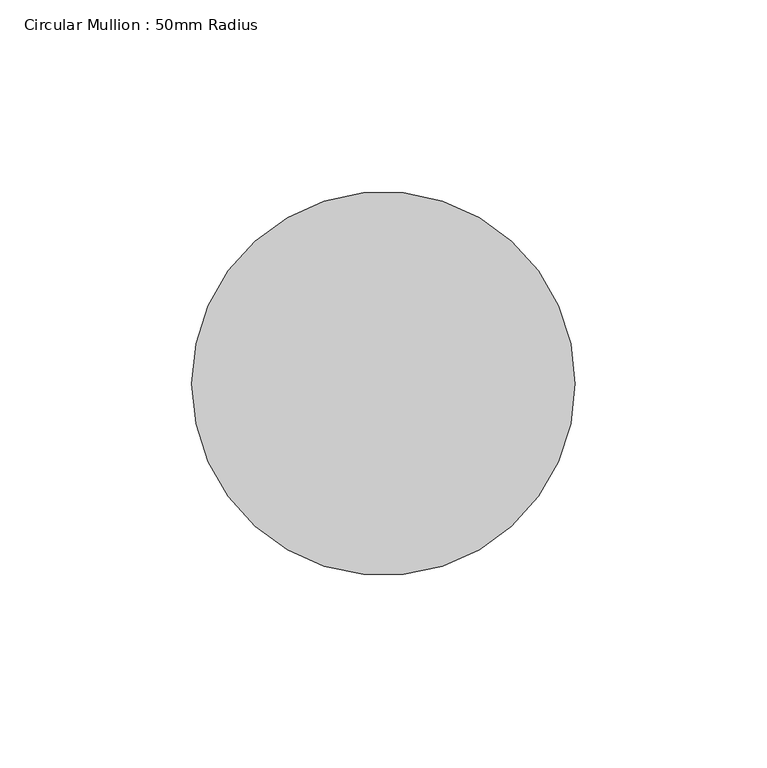
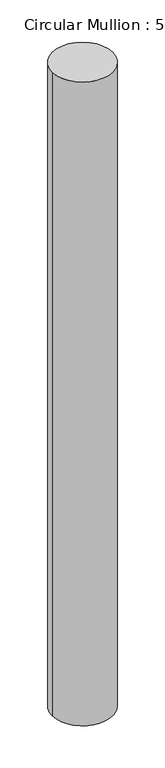
"""IFC4 building model written with IfcOpenShell, lengths in millimetres: member geometry, Circular Mullion : 50mm Radius."""

import ifcopenshell
import ifcopenshell.guid

model = None  # the IFC model being written
_history = None  # IfcOwnerHistory: only IFC2X3 demands one
_inside = {}  # id of a spatial element -> (the spatial element, [elements in it])
_under = {}  # id of a project, library or spatial element -> (it, [spatial elements below it])
_declared = {}  # id of a project -> (the project, [libraries it declares])
_typed = {}  # id of a type object -> (the type object, [elements of that type])
_made_of = {}  # id of a material, layer set ... -> (it, [elements and type objects made of it])


def new_model(schema):
    """Start an empty IFC model of exactly this schema.

    Asked for "IFC4X3", IfcOpenShell would pick the latest addendum, in which some entities
    have other attributes; the version numbers below select the first issue.
    IFC2X3 requires an IfcOwnerHistory on every rooted entity: one is made here for all.
    """
    global model, _history
    if schema == "IFC4X3":
        model = ifcopenshell.file(schema_version=(4, 3, 0, 0))
    else:
        model = ifcopenshell.file(schema=schema)
    _inside.clear()
    _under.clear()
    _declared.clear()
    _typed.clear()
    _made_of.clear()
    _history = None
    if model.schema == "IFC2X3":
        org = make("IfcOrganization", Name="unknown")
        user = make(
            "IfcPersonAndOrganization",
            ThePerson=make("IfcPerson", FamilyName="unknown"),
            TheOrganization=org,
        )
        app = make(
            "IfcApplication",
            ApplicationDeveloper=org,
            Version="unknown",
            ApplicationFullName="unknown",
            ApplicationIdentifier="unknown",
        )
        _history = make(
            "IfcOwnerHistory",
            OwningUser=user,
            OwningApplication=app,
            ChangeAction="ADDED",
            CreationDate=0,
        )
    return model


def make(cls, **values):
    """One entity of the class cls with the attributes given. An attribute that is None is left unset."""
    return model.create_entity(
        cls, **{name: value for name, value in values.items() if value is not None}
    )


def rooted(cls, **values):
    """An entity with a GlobalId (a new one), such as an element, a storey or a relation."""
    return make(cls, GlobalId=ifcopenshell.guid.new(), OwnerHistory=_history, **values)


def si_unit(unit_type, name, prefix=None):
    """IfcSIUnit, for example si_unit("LENGTHUNIT", "METRE", prefix="MILLI")."""
    return make("IfcSIUnit", UnitType=unit_type, Prefix=prefix, Name=name)


def assignment(units):
    """IfcUnitAssignment: the units of a project."""
    return None if units is None else make("IfcUnitAssignment", Units=units)


def point(xyz):
    """IfcCartesianPoint."""
    return None if xyz is None else make("IfcCartesianPoint", Coordinates=xyz)


def direction(xyz):
    """IfcDirection."""
    return None if xyz is None else make("IfcDirection", DirectionRatios=xyz)


def frame(location, z_axis=None, x_axis=None):
    """IfcAxis2Placement3D, a coordinate frame: its origin and axes. An axis left out is left unset."""
    return make(
        "IfcAxis2Placement3D",
        Location=point(location),
        Axis=direction(z_axis),
        RefDirection=direction(x_axis),
    )


def frame_2d(location, x_axis=None):
    """IfcAxis2Placement2D, a coordinate frame in the plane: its origin and x axis."""
    return make(
        "IfcAxis2Placement2D", Location=point(location), RefDirection=direction(x_axis)
    )


def origin():
    """The frame at (0, 0, 0) with its axes left unset."""
    return frame((0.0, 0.0, 0.0))


def origin_2d():
    """The frame at (0, 0) in the plane with its x axis left unset."""
    return frame_2d((0.0, 0.0))


def place(relative_to, where):
    """IfcLocalPlacement: puts the frame where relative to a parent placement (None: the world)."""
    return make(
        "IfcLocalPlacement", PlacementRelTo=relative_to, RelativePlacement=where
    )


def context(
    kind, dimensions, precision=None, world=None, true_north=None, identifier=None
):
    """IfcGeometricRepresentationContext, for example the 3D "Model" context."""
    return make(
        "IfcGeometricRepresentationContext",
        ContextIdentifier=identifier,
        ContextType=kind,
        CoordinateSpaceDimension=dimensions,
        Precision=precision,
        WorldCoordinateSystem=world,
        TrueNorth=true_north,
    )


def project(units=None, contexts=None):
    """IfcProject with its units and contexts."""
    return rooted(
        "IfcProject",
        Name="project",
        RepresentationContexts=contexts,
        UnitsInContext=assignment(units),
    )


def spatial(cls, under=None, at=None, **own):
    """A site, building, storey or space (cls), placed at a placement, below another one or the project."""
    s = rooted(cls, ObjectPlacement=at, **own)
    if under is not None:
        _under.setdefault(under.id(), (under, []))[1].append(s)
    return s


def circle_curve(where, radius):
    """IfcCircle in the frame where."""
    return make("IfcCircle", Position=where, Radius=radius)


def trimmed(basis, trim1, trim2, sense, master):
    """IfcTrimmedCurve: the piece of a basis curve between two trims."""
    return make(
        "IfcTrimmedCurve",
        BasisCurve=basis,
        Trim1=trim1,
        Trim2=trim2,
        SenseAgreement=sense,
        MasterRepresentation=master,
    )


def segment(curve, same_sense, transition):
    """IfcCompositeCurveSegment."""
    return make(
        "IfcCompositeCurveSegment",
        Transition=transition,
        SameSense=same_sense,
        ParentCurve=curve,
    )


def composite_curve(segments, self_intersect=None):
    """IfcCompositeCurve: segments joined end to end."""
    return make("IfcCompositeCurve", Segments=segments, SelfIntersect=self_intersect)


def outline(outer, holes=None, kind="AREA"):
    """IfcArbitraryClosedProfileDef: a profile drawn as a closed curve; with holes, ...WithVoids."""
    if holes is None:
        return make("IfcArbitraryClosedProfileDef", ProfileType=kind, OuterCurve=outer)
    return make(
        "IfcArbitraryProfileDefWithVoids",
        ProfileType=kind,
        OuterCurve=outer,
        InnerCurves=holes,
    )


def extrude(swept, where, along, depth):
    """IfcExtrudedAreaSolid: the profile swept, set in the frame where, extruded along a direction by depth."""
    return make(
        "IfcExtrudedAreaSolid",
        SweptArea=swept,
        Position=where,
        ExtrudedDirection=direction(along),
        Depth=depth,
    )


def shape(context_of_items, identifier, shape_type, items):
    """IfcShapeRepresentation: the items that make up one representation, for example the "Body"."""
    return make(
        "IfcShapeRepresentation",
        ContextOfItems=context_of_items,
        RepresentationIdentifier=identifier,
        RepresentationType=shape_type,
        Items=items,
    )


def source(mapping_origin, context_of_items, identifier, shape_type, items):
    """IfcRepresentationMap: a shape defined once, which mapped items show again and again."""
    return make(
        "IfcRepresentationMap",
        MappingOrigin=mapping_origin,
        MappedRepresentation=shape(context_of_items, identifier, shape_type, items),
    )


def transform(
    local_origin,
    x_axis=None,
    y_axis=None,
    z_axis=None,
    scale=None,
    scale2=None,
    scale3=None,
    uniform=True,
):
    """IfcCartesianTransformationOperator3D, or its non-uniform kind. x_axis, y_axis, z_axis: its Axis1, 2, 3."""
    if uniform:
        return make(
            "IfcCartesianTransformationOperator3D",
            Axis1=direction(x_axis),
            Axis2=direction(y_axis),
            LocalOrigin=point(local_origin),
            Scale=scale,
            Axis3=direction(z_axis),
        )
    return make(
        "IfcCartesianTransformationOperator3DnonUniform",
        Axis1=direction(x_axis),
        Axis2=direction(y_axis),
        LocalOrigin=point(local_origin),
        Scale=scale,
        Axis3=direction(z_axis),
        Scale2=scale2,
        Scale3=scale3,
    )


def mapped(mapping_source, mapping_target):
    """IfcMappedItem: shows the shape of a source again, moved by a transform."""
    return make(
        "IfcMappedItem", MappingSource=mapping_source, MappingTarget=mapping_target
    )


def made_of(thing, what):
    """Note that an element or type object is made of a material, layer set ...; save() writes the relation."""
    if what is not None:
        _made_of.setdefault(what.id(), (what, []))[1].append(thing)
    return thing


def element(
    cls,
    number,
    at=None,
    inside=None,
    cuts=None,
    type_object=None,
    material=None,
    context=None,
    identifier="Body",
    shape_type=None,
    held_by="IfcProductDefinitionShape",
    body=None,
    shapes=None,
    **own,
):
    """One element of the class cls, such as IfcWall. Its Tag is "e" and its number.

    at: its placement. inside: the storey or other place that contains it. cuts: it is an
    opening in that element (IfcRelVoidsElement). A single representation is given by context,
    identifier, shape_type and body (its items); several are given by shapes. held_by: the class
    of the entity that holds the representations. save() writes the other relations.
    """
    e = rooted(cls, Tag="e%d" % number, ObjectPlacement=at, **own)
    if body is not None:
        shapes = [shape(context, identifier, shape_type, body)]
    if shapes is not None:
        e.Representation = make(held_by, Representations=shapes)
    if inside is not None:
        _inside.setdefault(inside.id(), (inside, []))[1].append(e)
    if cuts is not None:
        rooted(
            "IfcRelVoidsElement", RelatingBuildingElement=cuts, RelatedOpeningElement=e
        )
    if type_object is not None:
        _typed.setdefault(type_object.id(), (type_object, []))[1].append(e)
    return made_of(e, material)


def aggregate(whole, parts):
    """IfcRelAggregates: a whole, such as a stair, and the parts it consists of."""
    return rooted("IfcRelAggregates", RelatingObject=whole, RelatedObjects=parts)


def save(model, path):
    """Write the relations noted so far, then the file.

    IfcRelAggregates (storeys below a building ...), IfcRelContainedInSpatialStructure (elements
    in a storey), IfcRelDefinesByType, IfcRelAssociatesMaterial and IfcRelDeclares: one each for
    every whole, place, type object, material and project.
    """
    for whole, parts in _under.values():
        aggregate(whole, parts)
    for where, things in _inside.values():
        rooted(
            "IfcRelContainedInSpatialStructure",
            RelatedElements=things,
            RelatingStructure=where,
        )
    for kind, things in _typed.values():
        rooted("IfcRelDefinesByType", RelatedObjects=things, RelatingType=kind)
    for what, things in _made_of.values():
        rooted("IfcRelAssociatesMaterial", RelatedObjects=things, RelatingMaterial=what)
    for by, libraries in _declared.values():
        rooted("IfcRelDeclares", RelatingContext=by, RelatedDefinitions=libraries)
    model.write(path)


def circular_mullion_50mm_radius_6861d0ce(model_context):
    return source(origin(), model_context, "Body", "SweptSolid", [
        extrude(outline(composite_curve([segment(trimmed(circle_curve(origin_2d(), 50.0), [point((50.0, 0.0))], [point((-50.0, 0.0))], False, "CARTESIAN"), True, "CONTINUOUS"), segment(trimmed(circle_curve(origin_2d(), 50.0), [point((-50.0, 0.0))], [point((50.0, 0.0))], False, "CARTESIAN"), True, "CONTINUOUS")], self_intersect=False)), frame((0.0, 0.0, -1128.4271566), z_axis=(0.0, 0.0, 1.0), x_axis=(1.0, 0.0, 0.0)), (0.0, 0.0, 1.0), 1128.4271566),
    ])


if __name__ == "__main__":
    model = new_model("IFC4")
    model_context = context("Model", 3, world=origin())
    ifc_project = project(units=[si_unit("LENGTHUNIT", "METRE", prefix="MILLI")], contexts=[model_context])
    site = spatial("IfcSite", under=ifc_project)
    building = spatial("IfcBuilding", under=site)
    placement = place(None, origin())
    circular_mullion_50mm_radius_shape = circular_mullion_50mm_radius_6861d0ce(model_context)
    element("IfcMember", 1, ObjectType="Circular Mullion : 50mm Radius", at=placement, inside=building, context=model_context, shape_type="MappedRepresentation", body=[
        mapped(circular_mullion_50mm_radius_shape, transform((0.0, 0.0, 0.0), x_axis=(1.0, 0.0, 0.0), y_axis=(0.0, 1.0, 0.0), z_axis=(0.0, 0.0, 1.0))),
    ])
    save(model, "model.ifc")

# Revit data of these elements
# Type "Circular Mullion : 50mm Radius"
#   built-in parameter 1007350 = 0.164042 (stored number, unit not read)
# Element 1 (IfcMember, "Circular Mullion : 50mm Radius")
#   Materials on its faces: "Aluminium"
# Materials
#   "Aluminium": class "Metal", colour RGB 247 247 247, transparency 0, Description = "Aluminium 6061", Cost = 0
